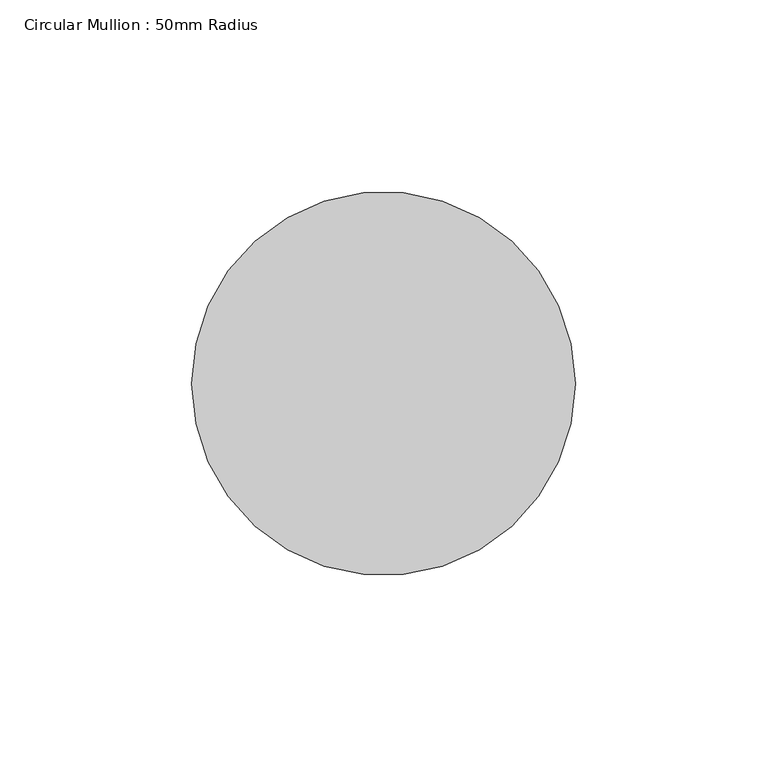
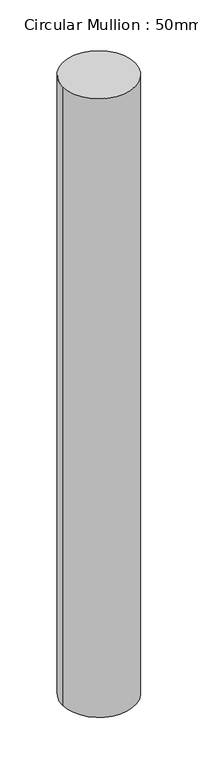
"""IFC4 building model written with IfcOpenShell, lengths in millimetres: member geometry, Circular Mullion : 50mm Radius."""

from ifc_helpers import new_model, si_unit, point, frame, origin, origin_2d, place, context, project, spatial, circle_curve, trimmed, segment, composite_curve, outline, extrude, source, transform, mapped, element, save


def circular_mullion_50mm_radius_c7ab1013(model_context):
    return source(origin(), model_context, "Body", "SweptSolid", [
        extrude(outline(composite_curve([segment(trimmed(circle_curve(origin_2d(), 50.0), [point((50.0, 0.0))], [point((-50.0, 0.0))], False, "CARTESIAN"), True, "CONTINUOUS"), segment(trimmed(circle_curve(origin_2d(), 50.0), [point((-50.0, 0.0))], [point((50.0, 0.0))], False, "CARTESIAN"), True, "CONTINUOUS")], self_intersect=False)), frame((0.0, 0.0, -901.8285359), z_axis=(0.0, 0.0, 1.0), x_axis=(1.0, 0.0, 0.0)), (0.0, 0.0, 1.0), 901.8285359),
    ])


if __name__ == "__main__":
    model = new_model("IFC4")
    model_context = context("Model", 3, world=origin())
    ifc_project = project(units=[si_unit("LENGTHUNIT", "METRE", prefix="MILLI")], contexts=[model_context])
    site = spatial("IfcSite", under=ifc_project)
    building = spatial("IfcBuilding", under=site)
    placement = place(None, origin())
    circular_mullion_50mm_radius_shape = circular_mullion_50mm_radius_c7ab1013(model_context)
    element("IfcMember", 1, ObjectType="Circular Mullion : 50mm Radius", at=placement, inside=building, context=model_context, shape_type="MappedRepresentation", body=[
        mapped(circular_mullion_50mm_radius_shape, transform((0.0, 0.0, 0.0), x_axis=(1.0, 0.0, 0.0), y_axis=(0.0, 1.0, 0.0), z_axis=(0.0, 0.0, 1.0))),
    ])
    save(model, "model.ifc")

# Revit data of these elements
# Type "Circular Mullion : 50mm Radius"
#   built-in parameter 1007350 = 0.164042 (stored number, unit not read)
# Element 1 (IfcMember, "Circular Mullion : 50mm Radius")
#   Materials on its faces: "Aluminium"
# Materials
#   "Aluminium": class "Metal", colour RGB 247 247 247, transparency 0, Description = "Aluminium 6061", Cost = 0
